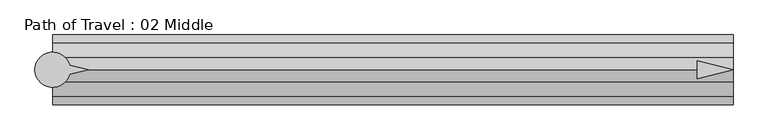
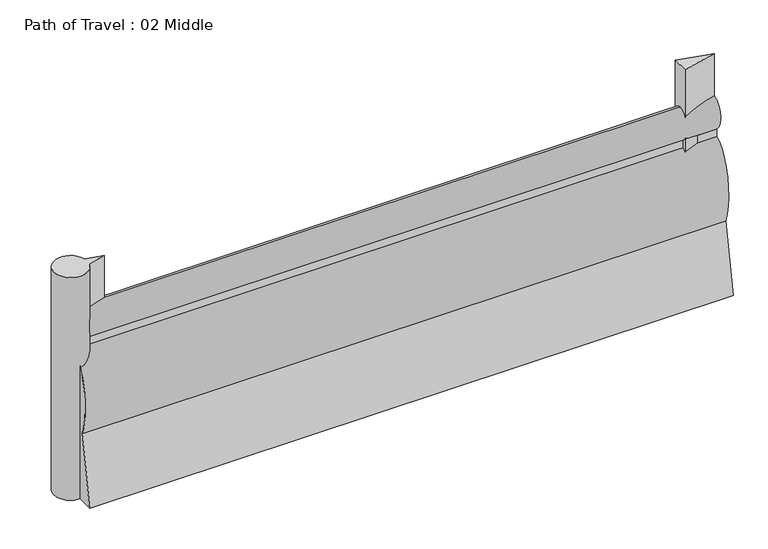
"""IFC4 building model written with IfcOpenShell, lengths in millimetres: proxy geometry, Path of Travel : 02 Middle."""

from ifc_helpers import new_model, si_unit, point, frame, frame_2d, origin, origin_with_axes, place, context, project, spatial, polyline, circle_curve, ellipse_curve, trimmed, segment, composite_curve, outline, extrude, source, transform, mapped, element, save
from ifc_brep_helpers import plane_surface, extruded_surface, advanced_brep


def path_of_travel_02_middle_5e5d3708(model_context):
    return source(origin(), model_context, "Body", "SolidModel", [
        advanced_brep(
        [(227.5554837, 0.0, 1727.2), (227.5554837, 42.9018657, 1436.6534209), (227.5554837, 42.9018657, 1363.4763406), (227.5554837, 184.1186263, 643.4144547), (227.5554837, 297.5699544, 0.0), (227.5554837, 145.6574193, 0.0), (227.5554837, 0.0, 584.2), (227.5554837, -145.6574193, 0.0), (227.5554837, -297.5699544, 0.0), (227.5554837, -184.1186263, 643.4144547), (227.5554837, -42.9018657, 1363.4763406), (227.5554837, -42.9018657, 1436.6534209), (6043.1050325, 0.0, 1727.2), (6043.1050325, -42.9018657, 1436.6534209), (6043.1050325, -42.9018657, 1363.4763406), (6043.1050325, -184.1186263, 643.4144547), (6043.1050325, -297.5699544, 0.0), (6043.1050325, -145.6574193, 0.0), (6043.1050325, 0.0, 584.2), (6043.1050325, 145.6574193, 0.0), (6043.1050325, 297.5699544, 0.0), (6043.1050325, 184.1186263, 643.4144547), (6043.1050325, 42.9018657, 1363.4763406), (6043.1050325, 42.9018657, 1436.6534209)],
        [
            (0, 1, ellipse_curve(frame((227.5554837, 0.0, 1574.8), z_axis=(-1.0, 0.0, 0.0), x_axis=(0.0, 0.0, 1.0)), 152.4, 101.6)),
            (1, 2),
            (2, 3, ellipse_curve(frame((227.5554837, 0.0, 914.4), z_axis=(-1.0, 0.0, 0.0), x_axis=(0.0, 0.0, -1.0)), 457.2, 228.6)),
            (3, 4),
            (4, 5),
            (5, 6),
            (6, 7),
            (7, 8),
            (8, 9),
            (9, 10, ellipse_curve(frame((227.5554837, 0.0, 914.4), z_axis=(-1.0, 0.0, 0.0), x_axis=(0.0, 0.0, -1.0)), 457.2, 228.6)),
            (10, 11),
            (11, 0, ellipse_curve(frame((227.5554837, 0.0, 1574.8), z_axis=(-1.0, 0.0, 0.0), x_axis=(0.0, 0.0, 1.0)), 152.4, 101.6)),
            (12, 13, ellipse_curve(frame((6043.1050325, 0.0, 1574.8), z_axis=(1.0, 0.0, 0.0), x_axis=(0.0, 0.0, 1.0)), 152.4, 101.6)),
            (13, 14),
            (14, 15, ellipse_curve(frame((6043.1050325, 0.0, 914.4), z_axis=(1.0, 0.0, 0.0), x_axis=(0.0, 0.0, -1.0)), 457.2, 228.6)),
            (15, 16),
            (16, 17),
            (17, 18),
            (18, 19),
            (19, 20),
            (20, 21),
            (21, 22, ellipse_curve(frame((6043.1050325, 0.0, 914.4), z_axis=(1.0, 0.0, 0.0), x_axis=(0.0, 0.0, -1.0)), 457.2, 228.6)),
            (22, 23),
            (23, 12, ellipse_curve(frame((6043.1050325, 0.0, 1574.8), z_axis=(1.0, 0.0, 0.0), x_axis=(0.0, 0.0, 1.0)), 152.4, 101.6)),
            (0, 12),
            (23, 1),
            (22, 2),
            (21, 3),
            (20, 4),
            (19, 5),
            (18, 6),
            (17, 7),
            (16, 8),
            (15, 9),
            (14, 10),
            (13, 11),
        ],
        [
            plane_surface(frame((227.5554837, 0.0, 0.0), z_axis=(-1.0, 0.0, 0.0), x_axis=(0.0, 0.0, 1.0))),
            plane_surface(frame((6043.1050325, 0.0, 0.0), z_axis=(1.0, 0.0, 0.0), x_axis=(0.0, 0.0, 1.0))),
            extruded_surface(trimmed(ellipse_curve(frame((6043.1050325, 0.0, 1574.8), z_axis=(-1.0, 0.0, 0.0), x_axis=(0.0, 0.0, 1.0)), 152.4, 101.6), [point((6043.1050325, 0.0, 1727.2))], [point((6043.1050325, 42.9018657, 1436.6534209))], True, "CARTESIAN"), (-5815.5495488, 0.0, 0.0), 5815.5495488),
            plane_surface(frame((227.5554837, 42.9018657, 1436.6534209), z_axis=(0.0, 1.0, 0.0), x_axis=(1.0, 0.0, 0.0))),
            extruded_surface(trimmed(ellipse_curve(frame((6043.1050325, 0.0, 914.4), z_axis=(-1.0, 0.0, 0.0), x_axis=(0.0, 0.0, -1.0)), 457.2, 228.6), [point((6043.1050325, 42.9018657, 1363.4763406))], [point((6043.1050325, 184.1186263, 643.4144547))], True, "CARTESIAN"), (-5815.5495488, 0.0, 0.0), 5815.5495488),
            plane_surface(frame((227.5554837, 184.1186263, 643.4144547), z_axis=(0.0, 0.9848077530122078, 0.1736481776669322), x_axis=(1.0, 0.0, 0.0))),
            plane_surface(frame((227.5554837, 297.5699544, 0.0), z_axis=(0.0, 0.0, -1.0), x_axis=(1.0, 0.0, 0.0))),
            plane_surface(frame((227.5554837, 145.6574193, 0.0), z_axis=(0.0, -0.9702957262760199, -0.2419218955995739), x_axis=(1.0, 0.0, 0.0))),
            plane_surface(frame((227.5554837, 0.0, 584.2), z_axis=(0.0, 0.9702957262759961, -0.24192189559966923), x_axis=(1.0, 0.0, 0.0))),
            plane_surface(frame((227.5554837, -145.6574193, 0.0), z_axis=(0.0, 0.0, -1.0), x_axis=(1.0, 0.0, 0.0))),
            plane_surface(frame((227.5554837, -297.5699544, 0.0), z_axis=(0.0, -0.984807753012208, 0.17364817766693066), x_axis=(1.0, 0.0, 0.0))),
            extruded_surface(trimmed(ellipse_curve(frame((6043.1050325, 0.0, 914.4), z_axis=(-1.0, 0.0, 0.0), x_axis=(0.0, 0.0, -1.0)), 457.2, 228.6), [point((6043.1050325, -184.1186263, 643.4144547))], [point((6043.1050325, -42.9018657, 1363.4763406))], True, "CARTESIAN"), (-5815.5495488, 0.0, 0.0), 5815.5495488),
            plane_surface(frame((227.5554837, -42.9018657, 1363.4763406), z_axis=(0.0, -1.0, 0.0), x_axis=(1.0, 0.0, 0.0))),
            extruded_surface(trimmed(ellipse_curve(frame((6043.1050325, 0.0, 1574.8), z_axis=(-1.0, 0.0, 0.0), x_axis=(0.0, 0.0, 1.0)), 152.4, 101.6), [point((6043.1050325, -42.9018657, 1436.6534209))], [point((6043.1050325, 0.0, 1727.2))], True, "CARTESIAN"), (-5815.5495488, 0.0, 0.0), 5815.5495488),
        ],
        [
            (0, [[1, 2, 3, 4, 5, 6, 7, 8, 9, 10, 11, 12]]),
            (1, [[13, 14, 15, 16, 17, 18, 19, 20, 21, 22, 23, 24]]),
            (2, [[-1, 25, -24, 26]]),
            (3, [[-2, -26, -23, 27]]),
            (4, [[-3, -27, -22, 28]]),
            (5, [[-4, -28, -21, 29]]),
            (6, [[-5, -29, -20, 30]]),
            (7, [[-6, -30, -19, 31]]),
            (8, [[-7, -31, -18, 32]]),
            (9, [[-8, -32, -17, 33]]),
            (10, [[-9, -33, -16, 34]]),
            (11, [[-10, -34, -15, 35]]),
            (12, [[-11, -35, -14, 36]]),
            (13, [[-12, -36, -13, -25]]),
        ],
    ),
        extrude(outline(polyline([(5737.0998859, 76.2006338), (6043.1050325, 0.0), (5737.0998859, -76.2006338), (5737.0998859, 76.2006338)])), origin_with_axes(), (0.0, 0.0, 1.0), 2129.5973753),
        extrude(outline(composite_curve([segment(polyline([(372.7837828, 39.4440225), (531.182385, 0.0), (372.7837828, -39.4440225)]), True, "CONTINUOUS"), segment(trimmed(circle_curve(frame_2d((227.2200886, 0.0)), 150.8131956), [point((372.7837828, -39.4440225))], [point((372.7837828, 39.4440225))], False, "CARTESIAN"), True, "CONTINUOUS")], self_intersect=False)), origin_with_axes(), (0.0, 0.0, 1.0), 2129.5973753),
    ])


if __name__ == "__main__":
    model = new_model("IFC4")
    model_context = context("Model", 3, world=origin())
    ifc_project = project(units=[si_unit("LENGTHUNIT", "METRE", prefix="MILLI")], contexts=[model_context])
    site = spatial("IfcSite", under=ifc_project)
    building = spatial("IfcBuilding", under=site)
    placement = place(None, origin())
    path_of_travel_02_middle_shape = path_of_travel_02_middle_5e5d3708(model_context)
    element("IfcBuildingElementProxy", 1, Name="Path of Travel : 02 Middle", ObjectType="Path of Travel : 02 Middle", at=placement, inside=building, context=model_context, shape_type="MappedRepresentation", body=[
        mapped(path_of_travel_02_middle_shape, transform((0.0, 0.0, 0.0), x_axis=(1.0, 0.0, 0.0), y_axis=(0.0, 1.0, 0.0), z_axis=(0.0, 0.0, 1.0))),
    ])
    save(model, "model.ifc")

# Revit data of these elements
# Type "Path of Travel : 02 Middle"
#   Path of Egress [instance default] = 4' - 0"
#   built-in parameter 1001306 [instance default] = 4 (stored number, unit not read)
#   Dot at Start = no
#   Arrow in Middle = yes
#   Arrow at End = no
#   Egress Path = none
# Element 1 (IfcBuildingElementProxy, "Path of Travel : 02 Middle")
#   Path of Egress = 19' - 0.95864"
#   built-in parameter 1001306 = 19.0799 (stored number, unit not read)
#   Materials on its faces: "Egress Path Solid", "solid"
# Materials
#   "Egress Path Solid": class "Unassigned", colour RGB 255 128 64, transparency 0.75, Comments = "Rendering appearance not upgraded "
#   "solid": class "Generic", colour RGB 120 120 120, transparency 0, Cost = 0
